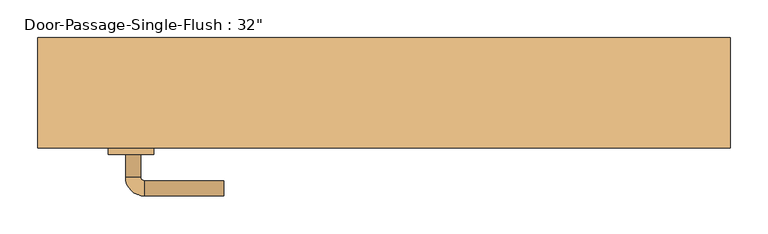
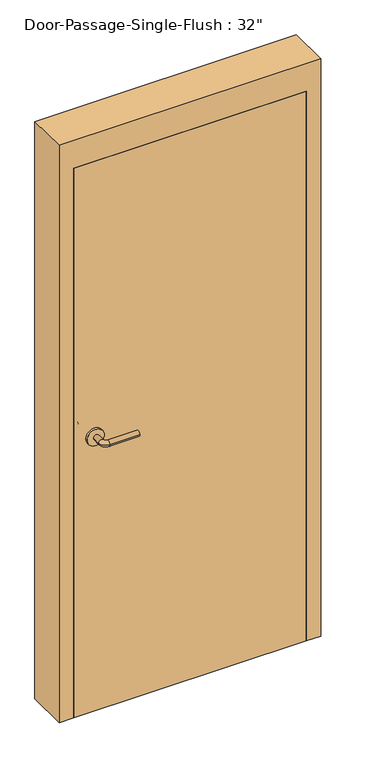
"""IFC4 building model written with IfcOpenShell, lengths in millimetres: door geometry."""

import ifcopenshell
import ifcopenshell.guid

model = None  # the IFC model being written
_history = None  # IfcOwnerHistory: only IFC2X3 demands one
_inside = {}  # id of a spatial element -> (the spatial element, [elements in it])
_under = {}  # id of a project, library or spatial element -> (it, [spatial elements below it])
_declared = {}  # id of a project -> (the project, [libraries it declares])
_typed = {}  # id of a type object -> (the type object, [elements of that type])
_made_of = {}  # id of a material, layer set ... -> (it, [elements and type objects made of it])


def new_model(schema):
    """Start an empty IFC model of exactly this schema.

    Asked for "IFC4X3", IfcOpenShell would pick the latest addendum, in which some entities
    have other attributes; the version numbers below select the first issue.
    IFC2X3 requires an IfcOwnerHistory on every rooted entity: one is made here for all.
    """
    global model, _history
    if schema == "IFC4X3":
        model = ifcopenshell.file(schema_version=(4, 3, 0, 0))
    else:
        model = ifcopenshell.file(schema=schema)
    _inside.clear()
    _under.clear()
    _declared.clear()
    _typed.clear()
    _made_of.clear()
    _history = None
    if model.schema == "IFC2X3":
        org = make("IfcOrganization", Name="unknown")
        user = make(
            "IfcPersonAndOrganization",
            ThePerson=make("IfcPerson", FamilyName="unknown"),
            TheOrganization=org,
        )
        app = make(
            "IfcApplication",
            ApplicationDeveloper=org,
            Version="unknown",
            ApplicationFullName="unknown",
            ApplicationIdentifier="unknown",
        )
        _history = make(
            "IfcOwnerHistory",
            OwningUser=user,
            OwningApplication=app,
            ChangeAction="ADDED",
            CreationDate=0,
        )
    return model


def make(cls, **values):
    """One entity of the class cls with the attributes given. An attribute that is None is left unset."""
    return model.create_entity(
        cls, **{name: value for name, value in values.items() if value is not None}
    )


def rooted(cls, **values):
    """An entity with a GlobalId (a new one), such as an element, a storey or a relation."""
    return make(cls, GlobalId=ifcopenshell.guid.new(), OwnerHistory=_history, **values)


def si_unit(unit_type, name, prefix=None):
    """IfcSIUnit, for example si_unit("LENGTHUNIT", "METRE", prefix="MILLI")."""
    return make("IfcSIUnit", UnitType=unit_type, Prefix=prefix, Name=name)


def assignment(units):
    """IfcUnitAssignment: the units of a project."""
    return None if units is None else make("IfcUnitAssignment", Units=units)


def point(xyz):
    """IfcCartesianPoint."""
    return None if xyz is None else make("IfcCartesianPoint", Coordinates=xyz)


def direction(xyz):
    """IfcDirection."""
    return None if xyz is None else make("IfcDirection", DirectionRatios=xyz)


def frame(location, z_axis=None, x_axis=None):
    """IfcAxis2Placement3D, a coordinate frame: its origin and axes. An axis left out is left unset."""
    return make(
        "IfcAxis2Placement3D",
        Location=point(location),
        Axis=direction(z_axis),
        RefDirection=direction(x_axis),
    )


def frame_2d(location, x_axis=None):
    """IfcAxis2Placement2D, a coordinate frame in the plane: its origin and x axis."""
    return make(
        "IfcAxis2Placement2D", Location=point(location), RefDirection=direction(x_axis)
    )


def origin():
    """The frame at (0, 0, 0) with its axes left unset."""
    return frame((0.0, 0.0, 0.0))


def origin_with_axes():
    """The frame at (0, 0, 0) with the z axis (0, 0, 1) and the x axis (1, 0, 0) written out."""
    return frame((0.0, 0.0, 0.0), z_axis=(0.0, 0.0, 1.0), x_axis=(1.0, 0.0, 0.0))


def place(relative_to, where):
    """IfcLocalPlacement: puts the frame where relative to a parent placement (None: the world)."""
    return make(
        "IfcLocalPlacement", PlacementRelTo=relative_to, RelativePlacement=where
    )


def context(
    kind, dimensions, precision=None, world=None, true_north=None, identifier=None
):
    """IfcGeometricRepresentationContext, for example the 3D "Model" context."""
    return make(
        "IfcGeometricRepresentationContext",
        ContextIdentifier=identifier,
        ContextType=kind,
        CoordinateSpaceDimension=dimensions,
        Precision=precision,
        WorldCoordinateSystem=world,
        TrueNorth=true_north,
    )


def project(units=None, contexts=None):
    """IfcProject with its units and contexts."""
    return rooted(
        "IfcProject",
        Name="project",
        RepresentationContexts=contexts,
        UnitsInContext=assignment(units),
    )


def spatial(cls, under=None, at=None, **own):
    """A site, building, storey or space (cls), placed at a placement, below another one or the project."""
    s = rooted(cls, ObjectPlacement=at, **own)
    if under is not None:
        _under.setdefault(under.id(), (under, []))[1].append(s)
    return s


def polyline(points):
    """IfcPolyline through the points."""
    return make("IfcPolyline", Points=[point(p) for p in points])


def circle_curve(where, radius):
    """IfcCircle in the frame where."""
    return make("IfcCircle", Position=where, Radius=radius)


def ellipse_curve(where, semi_axis1, semi_axis2):
    """IfcEllipse in the frame where."""
    return make(
        "IfcEllipse", Position=where, SemiAxis1=semi_axis1, SemiAxis2=semi_axis2
    )


def trimmed(basis, trim1, trim2, sense, master):
    """IfcTrimmedCurve: the piece of a basis curve between two trims."""
    return make(
        "IfcTrimmedCurve",
        BasisCurve=basis,
        Trim1=trim1,
        Trim2=trim2,
        SenseAgreement=sense,
        MasterRepresentation=master,
    )


def segment(curve, same_sense, transition):
    """IfcCompositeCurveSegment."""
    return make(
        "IfcCompositeCurveSegment",
        Transition=transition,
        SameSense=same_sense,
        ParentCurve=curve,
    )


def composite_curve(segments, self_intersect=None):
    """IfcCompositeCurve: segments joined end to end."""
    return make("IfcCompositeCurve", Segments=segments, SelfIntersect=self_intersect)


def outline(outer, holes=None, kind="AREA"):
    """IfcArbitraryClosedProfileDef: a profile drawn as a closed curve; with holes, ...WithVoids."""
    if holes is None:
        return make("IfcArbitraryClosedProfileDef", ProfileType=kind, OuterCurve=outer)
    return make(
        "IfcArbitraryProfileDefWithVoids",
        ProfileType=kind,
        OuterCurve=outer,
        InnerCurves=holes,
    )


def extrude(swept, where, along, depth):
    """IfcExtrudedAreaSolid: the profile swept, set in the frame where, extruded along a direction by depth."""
    return make(
        "IfcExtrudedAreaSolid",
        SweptArea=swept,
        Position=where,
        ExtrudedDirection=direction(along),
        Depth=depth,
    )


def faces_of(points, faces, orient=None, outer=None):
    """IfcFace entities. A face is a list of loops; a loop is a list of indices into points, from 0.

    orient and outer hold one flag for each loop. By default every Orientation is true, the
    first loop of a face is its IfcFaceOuterBound and the others are IfcFaceBound.
    """
    made = []
    for i, loops in enumerate(faces):
        bounds = []
        for j, loop in enumerate(loops):
            is_outer = j == 0 if outer is None else outer[i][j]
            bounds.append(
                make(
                    "IfcFaceOuterBound" if is_outer else "IfcFaceBound",
                    Bound=make("IfcPolyLoop", Polygon=[points[k] for k in loop]),
                    Orientation=True if orient is None else orient[i][j],
                )
            )
        made.append(make("IfcFace", Bounds=bounds))
    return made


def faceted_brep(points, faces, orient=None, outer=None, voids=None):
    """IfcFacetedBrep: a solid bounded by flat faces; with voids (closed shells), ...WithVoids."""
    shared = [point(p) for p in points]
    hull = make("IfcClosedShell", CfsFaces=faces_of(shared, faces, orient, outer))
    if voids is None:
        return make("IfcFacetedBrep", Outer=hull)
    return make(
        "IfcFacetedBrepWithVoids",
        Outer=hull,
        Voids=[
            make(cls, CfsFaces=faces_of(shared, fs, o, b)) for cls, fs, o, b in voids
        ],
    )


def shape(context_of_items, identifier, shape_type, items):
    """IfcShapeRepresentation: the items that make up one representation, for example the "Body"."""
    return make(
        "IfcShapeRepresentation",
        ContextOfItems=context_of_items,
        RepresentationIdentifier=identifier,
        RepresentationType=shape_type,
        Items=items,
    )


def source(mapping_origin, context_of_items, identifier, shape_type, items):
    """IfcRepresentationMap: a shape defined once, which mapped items show again and again."""
    return make(
        "IfcRepresentationMap",
        MappingOrigin=mapping_origin,
        MappedRepresentation=shape(context_of_items, identifier, shape_type, items),
    )


def transform(
    local_origin,
    x_axis=None,
    y_axis=None,
    z_axis=None,
    scale=None,
    scale2=None,
    scale3=None,
    uniform=True,
):
    """IfcCartesianTransformationOperator3D, or its non-uniform kind. x_axis, y_axis, z_axis: its Axis1, 2, 3."""
    if uniform:
        return make(
            "IfcCartesianTransformationOperator3D",
            Axis1=direction(x_axis),
            Axis2=direction(y_axis),
            LocalOrigin=point(local_origin),
            Scale=scale,
            Axis3=direction(z_axis),
        )
    return make(
        "IfcCartesianTransformationOperator3DnonUniform",
        Axis1=direction(x_axis),
        Axis2=direction(y_axis),
        LocalOrigin=point(local_origin),
        Scale=scale,
        Axis3=direction(z_axis),
        Scale2=scale2,
        Scale3=scale3,
    )


def mapped(mapping_source, mapping_target):
    """IfcMappedItem: shows the shape of a source again, moved by a transform."""
    return make(
        "IfcMappedItem", MappingSource=mapping_source, MappingTarget=mapping_target
    )


def made_of(thing, what):
    """Note that an element or type object is made of a material, layer set ...; save() writes the relation."""
    if what is not None:
        _made_of.setdefault(what.id(), (what, []))[1].append(thing)
    return thing


def element(
    cls,
    number,
    at=None,
    inside=None,
    cuts=None,
    type_object=None,
    material=None,
    context=None,
    identifier="Body",
    shape_type=None,
    held_by="IfcProductDefinitionShape",
    body=None,
    shapes=None,
    **own,
):
    """One element of the class cls, such as IfcWall. Its Tag is "e" and its number.

    at: its placement. inside: the storey or other place that contains it. cuts: it is an
    opening in that element (IfcRelVoidsElement). A single representation is given by context,
    identifier, shape_type and body (its items); several are given by shapes. held_by: the class
    of the entity that holds the representations. save() writes the other relations.
    """
    e = rooted(cls, Tag="e%d" % number, ObjectPlacement=at, **own)
    if body is not None:
        shapes = [shape(context, identifier, shape_type, body)]
    if shapes is not None:
        e.Representation = make(held_by, Representations=shapes)
    if inside is not None:
        _inside.setdefault(inside.id(), (inside, []))[1].append(e)
    if cuts is not None:
        rooted(
            "IfcRelVoidsElement", RelatingBuildingElement=cuts, RelatedOpeningElement=e
        )
    if type_object is not None:
        _typed.setdefault(type_object.id(), (type_object, []))[1].append(e)
    return made_of(e, material)


def aggregate(whole, parts):
    """IfcRelAggregates: a whole, such as a stair, and the parts it consists of."""
    return rooted("IfcRelAggregates", RelatingObject=whole, RelatedObjects=parts)


def save(model, path):
    """Write the relations noted so far, then the file.

    IfcRelAggregates (storeys below a building ...), IfcRelContainedInSpatialStructure (elements
    in a storey), IfcRelDefinesByType, IfcRelAssociatesMaterial and IfcRelDeclares: one each for
    every whole, place, type object, material and project.
    """
    for whole, parts in _under.values():
        aggregate(whole, parts)
    for where, things in _inside.values():
        rooted(
            "IfcRelContainedInSpatialStructure",
            RelatedElements=things,
            RelatingStructure=where,
        )
    for kind, things in _typed.values():
        rooted("IfcRelDefinesByType", RelatedObjects=things, RelatingType=kind)
    for what, things in _made_of.values():
        rooted("IfcRelAssociatesMaterial", RelatedObjects=things, RelatingMaterial=what)
    for by, libraries in _declared.values():
        rooted("IfcRelDeclares", RelatingContext=by, RelatedDefinitions=libraries)
    model.write(path)


def plane_surface(at):
    """IfcPlane: the flat surface through the origin of the frame at, square to its z axis."""
    return make("IfcPlane", Position=at)


def cylinder_surface(at, radius):
    """IfcCylindricalSurface: all points at the distance radius from the z axis of the frame at."""
    return make("IfcCylindricalSurface", Position=at, Radius=radius)


def revolved_surface(curve, axis_point, axis_direction):
    """IfcSurfaceOfRevolution: the curve turned about the line through axis_point along axis_direction."""
    return make(
        "IfcSurfaceOfRevolution",
        SweptCurve=make("IfcArbitraryOpenProfileDef", ProfileType="CURVE", Curve=curve),
        AxisPosition=make("IfcAxis1Placement", Location=point(axis_point), Axis=direction(axis_direction)),
    )


def advanced_brep(points, edges, surfaces, faces):
    """IfcAdvancedBrep: a solid bounded by faces that lie on surfaces and meet in shared edges.

    An edge is (start, end): straight between two places in points (the first is 0);
    or (start, end, curve); or (start, end, curve, False) where it runs against its curve.
    A face is (place in surfaces, loops), or (place, loops, False) where it looks against
    its surface's normal. A loop lists edges by number (the first is 1), with a minus sign
    where the edge is run from its end to its start. The first loop is the outer one.
    """
    corners = [point(p) for p in points]
    vertices = [make("IfcVertexPoint", VertexGeometry=c) for c in corners]
    made = []
    for start, end, *more in edges:
        made.append(
            make(
                "IfcEdgeCurve",
                EdgeStart=vertices[start],
                EdgeEnd=vertices[end],
                EdgeGeometry=more[0] if more else make("IfcPolyline", Points=[corners[start], corners[end]]),
                SameSense=more[1] if len(more) > 1 else True,
            )
        )
    hull = []
    for where, loops, *sense in faces:
        bounds = []
        for j, loop in enumerate(loops):
            ring = [make("IfcOrientedEdge", EdgeElement=made[abs(k) - 1], Orientation=k > 0) for k in loop]
            bounds.append(
                make(
                    "IfcFaceOuterBound" if j == 0 else "IfcFaceBound",
                    Bound=make("IfcEdgeLoop", EdgeList=ring),
                    Orientation=True,
                )
            )
        hull.append(make("IfcAdvancedFace", Bounds=bounds, FaceSurface=surfaces[where], SameSense=sense[0] if sense else True))
    return make("IfcAdvancedBrep", Outer=make("IfcClosedShell", CfsFaces=hull))


def door_95bf5518(model_context):
    return source(origin(), model_context, "Body", "SolidModel", [
        advanced_brep(
        [(-341.390625, 11.175, 1016.0), (-321.390625, 11.175, 1016.0), (-341.390625, 41.175, 1016.0), (-321.390625, 41.175, 1016.0), (-316.390625, 46.175, 1016.0), (-316.390625, 66.175, 1016.0), (-211.390625, 66.175, 1016.0), (-211.390625, 46.175, 1016.0)],
        [
            (0, 1, circle_curve(frame((-331.390625, 11.175, 1016.0), z_axis=(0.0, -1.0, 0.0), x_axis=(1.0, 0.0, 0.0)), 10.0)),
            (1, 0, circle_curve(frame((-331.390625, 11.175, 1016.0), z_axis=(0.0, -1.0, 0.0), x_axis=(1.0, 0.0, 0.0)), 10.0)),
            (0, 2),
            (2, 3, circle_curve(frame((-331.390625, 41.175, 1016.0), z_axis=(0.0, -1.0, 0.0), x_axis=(1.0, 0.0, 0.0)), 10.0)),
            (3, 1),
            (3, 2, circle_curve(frame((-331.390625, 41.175, 1016.0), z_axis=(0.0, -1.0, 0.0), x_axis=(1.0, 0.0, 0.0)), 10.0)),
            (4, 3, circle_curve(frame((-316.390625, 41.175, 1016.0), z_axis=(0.0, 0.0, 1.0), x_axis=(-1.0, 0.0, 0.0)), 5.0)),
            (2, 5, circle_curve(frame((-316.390625, 41.175, 1016.0), z_axis=(0.0, 0.0, -1.0), x_axis=(-1.0, 0.0, 0.0)), 25.0)),
            (5, 4, circle_curve(frame((-316.390625, 56.175, 1016.0), z_axis=(-1.0, 0.0, 0.0), x_axis=(0.0, -1.0, 0.0)), 10.0)),
            (4, 5, circle_curve(frame((-316.390625, 56.175, 1016.0), z_axis=(-1.0, 0.0, 0.0), x_axis=(0.0, -1.0, 0.0)), 10.0)),
            (6, 7, circle_curve(frame((-211.390625, 56.175, 1016.0), z_axis=(1.0, 0.0, 0.0), x_axis=(0.0, -1.0, 0.0)), 10.0)),
            (7, 6, circle_curve(frame((-211.390625, 56.175, 1016.0), z_axis=(1.0, 0.0, 0.0), x_axis=(0.0, -1.0, 0.0)), 10.0)),
            (5, 6),
            (7, 4),
        ],
        [
            plane_surface(frame((-331.390625, 11.175, 1016.0), z_axis=(0.0, -1.0, 0.0), x_axis=(0.0, 0.0, 1.0))),
            cylinder_surface(frame((-331.390625, 11.175, 1016.0), z_axis=(0.0, -1.0, 0.0), x_axis=(1.0, 0.0, 0.0)), 10.0),
            revolved_surface(trimmed(ellipse_curve(frame((-331.390625, 41.175, 1016.0), z_axis=(0.0, -1.0, 0.0), x_axis=(1.0, 0.0, 0.0)), 10.0, 10.0), [point((-341.390625, 41.175, 1016.0))], [point((-321.390625, 41.175, 1016.0))], True, "CARTESIAN"), (-316.390625, 41.175, 1016.0), (0.0, 0.0, -1.0)),
            revolved_surface(trimmed(ellipse_curve(frame((-331.390625, 41.175, 1016.0), z_axis=(0.0, -1.0, 0.0), x_axis=(1.0, 0.0, 0.0)), 10.0, 10.0), [point((-321.390625, 41.175, 1016.0))], [point((-341.390625, 41.175, 1016.0))], True, "CARTESIAN"), (-316.390625, 41.175, 1016.0), (0.0, 0.0, -1.0)),
            plane_surface(frame((-211.390625, 56.175, 1016.0), z_axis=(1.0, 0.0, 0.0), x_axis=(0.0, 0.0, 1.0))),
            cylinder_surface(frame((-316.390625, 56.175, 1016.0), z_axis=(-1.0, 0.0, 0.0), x_axis=(0.0, -1.0, 0.0)), 10.0),
        ],
        [
            (0, [[1, 2]]),
            (1, [[-1, 3, 4, 5]]),
            (1, [[-2, -5, 6, -3]]),
            (2, [[7, -4, 8, 9]]),
            (3, [[-8, -6, -7, 10]]),
            (4, [[11, 12]]),
            (5, [[-9, 13, -12, 14]]),
            (5, [[-10, -14, -11, -13]]),
        ],
    ),
        extrude(outline(composite_curve([segment(trimmed(circle_curve(frame_2d((1016.0, -333.890625)), 30.0), [point((1016.0, -363.890625))], [point((1016.0, -303.890625))], False, "CARTESIAN"), True, "CONTINUOUS"), segment(trimmed(circle_curve(frame_2d((1016.0, -333.890625)), 30.0), [point((1016.0, -303.890625))], [point((1016.0, -363.890625))], False, "CARTESIAN"), True, "CONTINUOUS")], self_intersect=False)), frame((0.0, 3.175, 0.0), z_axis=(0.0, 1.0, 0.0), x_axis=(0.0, 0.0, 1.0)), (0.0, 0.0, 1.0), 8.0),
        advanced_brep(
        [(-341.390625, -49.275, 1016.0), (-321.390625, -49.275, 1016.0), (-321.390625, -79.275, 1016.0), (-341.390625, -79.275, 1016.0), (-316.390625, -84.275, 1016.0), (-316.390625, -104.275, 1016.0), (-211.390625, -104.275, 1016.0), (-211.390625, -84.275, 1016.0)],
        [
            (0, 1, circle_curve(frame((-331.390625, -49.275, 1016.0), z_axis=(0.0, 1.0, 0.0), x_axis=(1.0, 0.0, 0.0)), 10.0)),
            (1, 0, circle_curve(frame((-331.390625, -49.275, 1016.0), z_axis=(0.0, 1.0, 0.0), x_axis=(1.0, 0.0, 0.0)), 10.0)),
            (1, 2),
            (2, 3, circle_curve(frame((-331.390625, -79.275, 1016.0), z_axis=(0.0, 1.0, 0.0), x_axis=(1.0, 0.0, 0.0)), 10.0)),
            (3, 0),
            (3, 2, circle_curve(frame((-331.390625, -79.275, 1016.0), z_axis=(0.0, 1.0, 0.0), x_axis=(1.0, 0.0, 0.0)), 10.0)),
            (4, 5, circle_curve(frame((-316.390625, -94.275, 1016.0), z_axis=(-1.0, 0.0, 0.0), x_axis=(0.0, 1.0, 0.0)), 10.0)),
            (5, 3, circle_curve(frame((-316.390625, -79.275, 1016.0), z_axis=(0.0, 0.0, -1.0), x_axis=(-1.0, 0.0, 0.0)), 25.0)),
            (2, 4, circle_curve(frame((-316.390625, -79.275, 1016.0), z_axis=(0.0, 0.0, 1.0), x_axis=(-1.0, 0.0, 0.0)), 5.0)),
            (5, 4, circle_curve(frame((-316.390625, -94.275, 1016.0), z_axis=(-1.0, 0.0, 0.0), x_axis=(0.0, 1.0, 0.0)), 10.0)),
            (6, 7, circle_curve(frame((-211.390625, -94.275, 1016.0), z_axis=(1.0, 0.0, 0.0), x_axis=(0.0, 1.0, 0.0)), 10.0)),
            (7, 6, circle_curve(frame((-211.390625, -94.275, 1016.0), z_axis=(1.0, 0.0, 0.0), x_axis=(0.0, 1.0, 0.0)), 10.0)),
            (4, 7),
            (6, 5),
        ],
        [
            plane_surface(frame((-331.390625, -49.275, 1016.0), z_axis=(0.0, 1.0, 0.0), x_axis=(0.0, 0.0, 1.0))),
            cylinder_surface(frame((-331.390625, -49.275, 1016.0), z_axis=(0.0, 1.0, 0.0), x_axis=(1.0, 0.0, 0.0)), 10.0),
            revolved_surface(trimmed(ellipse_curve(frame((-331.390625, -79.275, 1016.0), z_axis=(0.0, -1.0, 0.0), x_axis=(1.0, 0.0, 0.0)), 10.0, 10.0), [point((-341.390625, -79.275, 1016.0))], [point((-321.390625, -79.275, 1016.0))], True, "CARTESIAN"), (-316.390625, -79.275, 1016.0), (0.0, 0.0, -1.0)),
            revolved_surface(trimmed(ellipse_curve(frame((-331.390625, -79.275, 1016.0), z_axis=(0.0, -1.0, 0.0), x_axis=(1.0, 0.0, 0.0)), 10.0, 10.0), [point((-321.390625, -79.275, 1016.0))], [point((-341.390625, -79.275, 1016.0))], True, "CARTESIAN"), (-316.390625, -79.275, 1016.0), (0.0, 0.0, -1.0)),
            plane_surface(frame((-211.390625, -94.275, 1016.0), z_axis=(1.0, 0.0, 0.0), x_axis=(0.0, 0.0, 1.0))),
            cylinder_surface(frame((-316.390625, -94.275, 1016.0), z_axis=(-1.0, 0.0, 0.0), x_axis=(0.0, 1.0, 0.0)), 10.0),
        ],
        [
            (0, [[1, 2]]),
            (1, [[3, 4, 5, -2]]),
            (1, [[-5, 6, -3, -1]]),
            (2, [[7, 8, -4, 9]]),
            (3, [[10, -9, -6, -8]]),
            (4, [[11, 12]]),
            (5, [[13, -11, 14, -7]]),
            (5, [[-14, -12, -13, -10]]),
        ],
    ),
        extrude(outline(composite_curve([segment(trimmed(circle_curve(frame_2d((1016.0, -333.890625)), 30.0), [point((1016.0, -363.890625))], [point((1016.0, -303.890625))], False, "CARTESIAN"), True, "CONTINUOUS"), segment(trimmed(circle_curve(frame_2d((1016.0, -333.890625)), 30.0), [point((1016.0, -303.890625))], [point((1016.0, -363.890625))], False, "CARTESIAN"), True, "CONTINUOUS")], self_intersect=False)), frame((0.0, -49.275, 0.0), z_axis=(0.0, 1.0, 0.0), x_axis=(0.0, 0.0, 1.0)), (0.0, 0.0, 1.0), 8.0),
        faceted_brep([(406.4, 7.9375, 0.0), (390.525, 7.9375, 0.0), (390.525, 55.5625, 0.0), (406.4, 55.5625, 0.0), (406.4, 104.775, 0.0), (457.2, 104.775, 0.0), (457.2, -41.275, 0.0), (406.4, -41.275, 0.0), (406.4, -41.275, 2032.0), (406.4, 7.9375, 2032.0), (457.2, -41.275, 2133.6), (-457.2, -41.275, 2133.6), (-457.2, -41.275, 0.0), (-406.4, -41.275, 0.0), (-406.4, -41.275, 2032.0), (457.2, 104.775, 2133.6), (406.4, 104.775, 2032.0), (-406.4, 104.775, 2032.0), (-406.4, 104.775, 0.0), (-457.2, 104.775, 0.0), (-457.2, 104.775, 2133.6), (406.4, 55.5625, 2032.0), (390.525, 55.5625, 2016.125), (-390.525, 55.5625, 2016.125), (-390.525, 55.5625, 0.0), (-406.4, 55.5625, 0.0), (-406.4, 55.5625, 2032.0), (390.525, 7.9375, 2016.125), (-406.4, 7.9375, 2032.0), (-406.4, 7.9375, 0.0), (-390.525, 7.9375, 0.0), (-390.525, 7.9375, 2016.125)], [[[0, 1, 2, 3, 4, 5, 6, 7]], [[7, 8, 9, 0]], [[6, 10, 11, 12, 13, 14, 8, 7]], [[5, 15, 10, 6]], [[4, 16, 17, 18, 19, 20, 15, 5]], [[3, 21, 16, 4]], [[2, 22, 23, 24, 25, 26, 21, 3]], [[1, 27, 22, 2]], [[0, 9, 28, 29, 30, 31, 27, 1]], [[8, 14, 28, 9]], [[16, 21, 26, 17]], [[22, 27, 31, 23]], [[12, 19, 18, 25, 24, 30, 29, 13]], [[13, 29, 28, 14]], [[11, 20, 19, 12]], [[17, 26, 25, 18]], [[23, 31, 30, 24]], [[15, 20, 11, 10]]]),
        extrude(outline(polyline([(406.4, 3.175), (406.4, -41.275), (-406.4, -41.275), (-406.4, 3.175), (406.4, 3.175)])), origin_with_axes(), (0.0, 0.0, 1.0), 2032.0),
    ])


if __name__ == "__main__":
    model = new_model("IFC4")
    model_context = context("Model", 3, world=origin())
    ifc_project = project(units=[si_unit("LENGTHUNIT", "METRE", prefix="MILLI")], contexts=[model_context])
    site = spatial("IfcSite", under=ifc_project)
    building = spatial("IfcBuilding", under=site)
    placement = place(None, origin())
    door_shape = door_95bf5518(model_context)
    element("IfcDoor", 1, ObjectType="Door-Passage-Single-Flush : 32\"", at=placement, inside=building, context=model_context, shape_type="MappedRepresentation", body=[
        mapped(door_shape, transform((0.0, 0.0, 0.0), x_axis=(1.0, 0.0, 0.0), y_axis=(0.0, 1.0, 0.0), z_axis=(0.0, 0.0, 1.0))),
    ])
    save(model, "model.ifc")

# Revit data of these elements
# Type "Door-Passage-Single-Flush : 32\""
#   Type Mark = "D10"
#   Assembly Code = "B2030200"
#   Analytic Construction = "Wooden"
#   Thickness = 0' - 1 3/4"
#   Thermal Resistance (R) = 0.455703 (m²·K)/W
#   Swing Angle [instance default] = 90.00°
#   Strike Height = 3' - 4"
#   Rough Width [instance default] = 3' - 0"
#   Rough Height [instance default] = 7' - 0"
#   MF Opening Height [instance default] = 0' - 4"
#   MF Opening Width [instance default] = 0' - 4"
#   Inset Calculate [instance default] = 0' - 4"
#   Masonry Inset [instance default] = 0' - 1"
#   Height = 6' - 8"
#   Width = 2' - 8"
#   Heat Transfer Coefficient (U) = 2.19465 W/(m²·K)
#   Masonry Frame Depth = 0' - 5 3/4"
#   Masonry Frame [instance default] = yes
#   Function = 1
#   Dry Wall Frame [instance default] = no
#   Panel Material = Wood - Birch
#   Frame Material = Metal - Paint Finish - Grey
#   Door Handle Material = Aluminum
#   Visual Light Transmittance = 0
#   Solar Heat Gain Coefficient = 0
#   Wall Closure = (empty or 0)
# Element 1 (IfcDoor, "Door-Passage-Single-Flush : 32\"")
#   Materials on its faces: "Aluminum", "Metal - Paint Finish - Grey", "Wood - Birch"
# Materials
#   "Wood - Birch": class "Wood", colour RGB 166 116 52, transparency 0, Cost = 0
#   "Metal - Paint Finish - Grey": class "Paint", colour RGB 104 104 104, transparency 0, Cost = 0
#   "Aluminum": class "Metal", colour RGB 247 247 247, transparency 0, Description = "Aluminum 6061", Cost = 0
